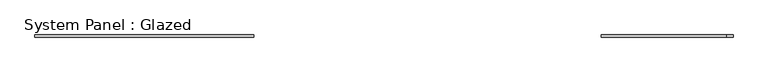
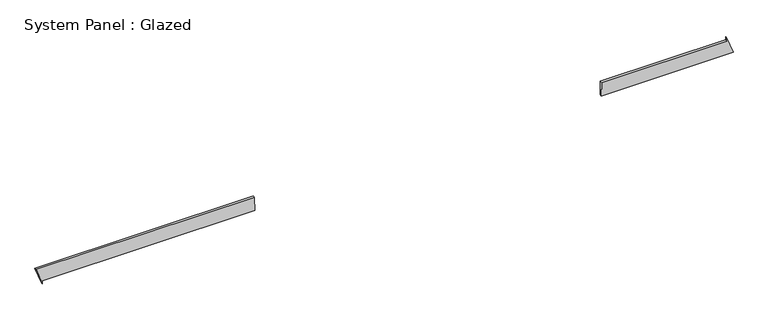
"""IFC4 building model written with IfcOpenShell, lengths in millimetres: plate geometry, System Panel : Glazed."""

from ifc_helpers import new_model, si_unit, frame, origin, place, context, project, spatial, polyline, outline, extrude, source, transform, mapped, element, save


def system_panel_glazed_28245ad9(model_context):
    return source(origin(), model_context, "Body", "SweptSolid", [
        extrude(outline(polyline([(35.3553391, 2505.7968783), (35.3553391, 4027.3319665), (234.8589574, 3956.5179694), (199.5036184, 3956.5175852), (199.5193516, 2508.4843015), (35.3553391, 2505.7968783)])), frame((0.0, -49.5, 0.0), z_axis=(0.0, 1.0, 0.0), x_axis=(0.0, 0.0, 1.0)), (0.0, 0.0, 1.0), 25.0),
        extrude(outline(polyline([(0.0, -3956.7216602), (35.3553391, -3956.7216602), (35.3553391, -1502.8981059), (199.5629538, -1504.5128119), (199.5903648, -4027.3319665), (0.0, -3956.7216602)])), frame((0.0, -49.5, 0.0), z_axis=(0.0, 1.0, 0.0), x_axis=(0.0, 0.0, 1.0)), (0.0, 0.0, 1.0), 25.0),
    ])


if __name__ == "__main__":
    model = new_model("IFC4")
    model_context = context("Model", 3, world=origin())
    ifc_project = project(units=[si_unit("LENGTHUNIT", "METRE", prefix="MILLI")], contexts=[model_context])
    site = spatial("IfcSite", under=ifc_project)
    building = spatial("IfcBuilding", under=site)
    placement = place(None, origin())
    system_panel_glazed_shape = system_panel_glazed_28245ad9(model_context)
    element("IfcPlate", 1, ObjectType="System Panel : Glazed", at=placement, inside=building, context=model_context, shape_type="MappedRepresentation", body=[
        mapped(system_panel_glazed_shape, transform((0.0, 0.0, 0.0), x_axis=(1.0, 0.0, 0.0), y_axis=(0.0, 1.0, 0.0), z_axis=(0.0, 0.0, 1.0))),
    ])
    save(model, "model.ifc")

# Revit data of these elements
# Element 1 (IfcPlate, "System Panel : Glazed")
#   Materials on its faces: "Glass"
# Materials
#   "Glass": class "Glass", colour RGB 218 227 224, transparency 0.85, Description = "Soda Lime Glass", Cost = 0
